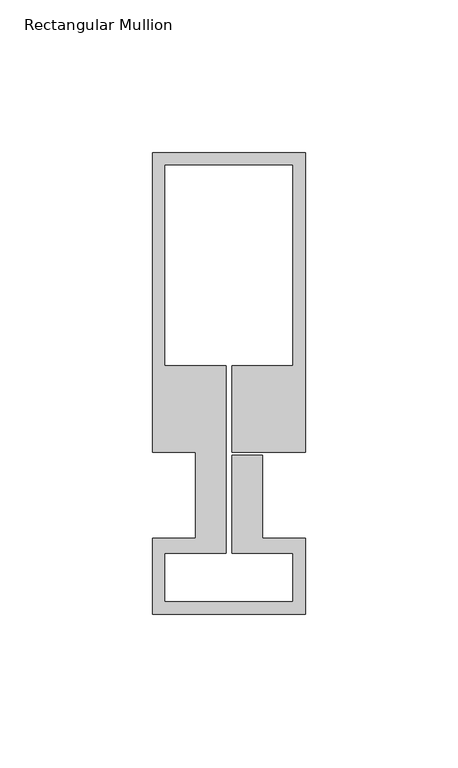
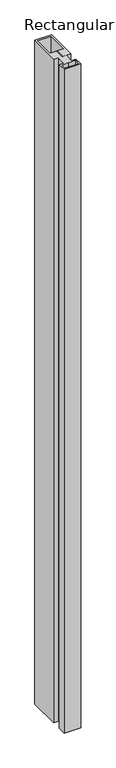
"""IFC4 building model written with IfcOpenShell, lengths in millimetres: member geometry, Rectangular Mullion : Schueco_FWS-50-HI_Mull_CovCap-20mm_Mull-85mm."""

from ifc_helpers import new_model, si_unit, frame, origin, place, context, project, spatial, polyline, outline, extrude, source, transform, mapped, element, save


def rectangular_mullion_bb2242ce(model_context):
    return source(origin(), model_context, "Body", "SweptSolid", [
        extrude(outline(polyline([(-50.0, 126.0), (0.0, 126.0), (0.0, 28.0), (-24.0, 28.0), (-24.0, 56.3), (-4.0, 56.3), (-4.0, 122.0), (-46.0, 122.0), (-46.0, 56.3), (-26.0, 56.3), (-26.0, -5.0), (-46.0, -5.0), (-46.0, -21.0), (-4.0, -21.0), (-4.0, -5.0), (-24.0, -5.0), (-24.0, 27.0), (-14.0, 27.0), (-14.0, -0.1), (0.0, -0.1), (0.0, -25.0), (-50.0, -25.0), (-50.0, -0.1), (-36.0, -0.1), (-36.0, 28.0), (-50.0, 28.0), (-50.0, 126.0)])), frame((0.0, 0.0, -2100.0), z_axis=(0.0, 0.0, 1.0), x_axis=(1.0, 0.0, 0.0)), (0.0, 0.0, 1.0), 2100.0),
    ])


if __name__ == "__main__":
    model = new_model("IFC4")
    model_context = context("Model", 3, world=origin())
    ifc_project = project(units=[si_unit("LENGTHUNIT", "METRE", prefix="MILLI")], contexts=[model_context])
    site = spatial("IfcSite", under=ifc_project)
    building = spatial("IfcBuilding", under=site)
    placement = place(None, origin())
    rectangular_mullion_shape = rectangular_mullion_bb2242ce(model_context)
    element("IfcMember", 1, ObjectType="Rectangular Mullion : Schueco_FWS-50-HI_Mull_CovCap-20mm_Mull-85mm", at=placement, inside=building, context=model_context, shape_type="MappedRepresentation", body=[
        mapped(rectangular_mullion_shape, transform((0.0, 0.0, 0.0), x_axis=(1.0, 0.0, 0.0), y_axis=(0.0, 1.0, 0.0), z_axis=(0.0, 0.0, 1.0))),
    ])
    save(model, "model.ifc")

# Revit data of these elements
# Type "Rectangular Mullion : Schueco_FWS-50-HI_Mull_CovCap-20mm_Mull-85mm"
#   Model = "FWS 50.HI"
#   Manufacturer = "Schueco International KG"
#   Type Comments = "Mullion"
#   Schueco thermal insulation standard = "Highly thermally insulated"
#   Burglar resistance = "RC 3"
#   Thermal insulation = "to 0.90 W/(m²K)"
#   built-in parameter 1007322 = 0.495407 (stored number, unit not read)
#   built-in parameter 1007321 = 0.0360892 (stored number, unit not read)
#   built-in parameter 1007320 = 0.0360892 (stored number, unit not read)
# Element 1 (IfcMember, "Rectangular Mullion : Schueco_FWS-50-HI_Mull_CovCap-20mm_Mull-85mm")
#   Materials on its faces: "Alu"
# Materials
#   "Alu": class "Glas", colour RGB 140 140 140, transparency 0
